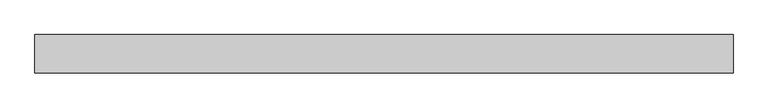
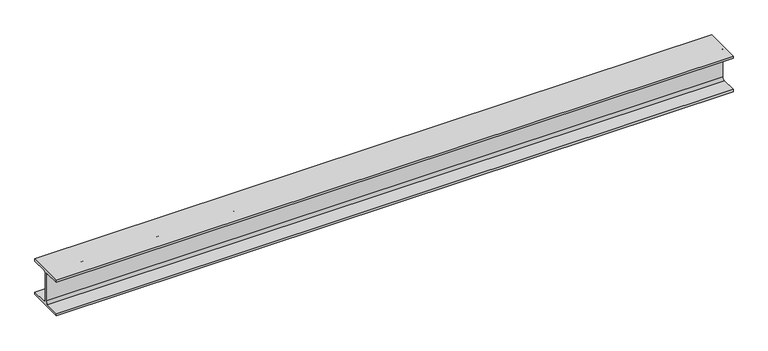
"""IFC4 building model written with IfcOpenShell, lengths in millimetres: beam geometry, 0912_Steel Framing_H-KSD3502 : H_SB_ASB_H-200x200x8x12."""

from ifc_helpers import new_model, si_unit, point, frame, frame_2d, origin, place, context, project, spatial, polyline, circle_curve, trimmed, segment, composite_curve, outline, extrude, source, transform, mapped, element, save


def beam_8723a7d4(model_context):
    return source(origin(), model_context, "Body", "SweptSolid", [
        extrude(outline(composite_curve([segment(polyline([(100.0, -88.0), (100.0, -100.0), (-100.0, -100.0), (-100.0, -88.0), (-17.0, -88.0)]), True, "CONTINUOUS"), segment(trimmed(circle_curve(frame_2d((-17.0, -75.0)), 13.0), [point((-17.0, -88.0))], [point((-4.0, -75.0))], True, "CARTESIAN"), True, "CONTINUOUS"), segment(polyline([(-4.0, -75.0), (-4.0, 75.0)]), True, "CONTINUOUS"), segment(trimmed(circle_curve(frame_2d((-17.0, 75.0)), 13.0), [point((-4.0, 75.0))], [point((-17.0, 88.0))], True, "CARTESIAN"), True, "CONTINUOUS"), segment(polyline([(-17.0, 88.0), (-100.0, 88.0), (-100.0, 100.0), (100.0, 100.0), (100.0, 88.0), (17.0, 88.0)]), True, "CONTINUOUS"), segment(trimmed(circle_curve(frame_2d((17.0, 75.0)), 13.0), [point((17.0, 88.0))], [point((4.0, 75.0))], True, "CARTESIAN"), True, "CONTINUOUS"), segment(polyline([(4.0, 75.0), (4.0, -75.0)]), True, "CONTINUOUS"), segment(trimmed(circle_curve(frame_2d((17.0, -75.0)), 13.0), [point((4.0, -75.0))], [point((17.0, -88.0))], True, "CARTESIAN"), True, "CONTINUOUS"), segment(polyline([(17.0, -88.0), (100.0, -88.0)]), True, "CONTINUOUS")], self_intersect=False)), frame((-1780.1436483, 0.0, 0.0), z_axis=(1.0, 0.0, 0.0), x_axis=(0.0, 1.0, 0.0)), (0.0, 0.0, 1.0), 3630.9979746),
    ])


if __name__ == "__main__":
    model = new_model("IFC4")
    model_context = context("Model", 3, world=origin())
    ifc_project = project(units=[si_unit("LENGTHUNIT", "METRE", prefix="MILLI")], contexts=[model_context])
    site = spatial("IfcSite", under=ifc_project)
    building = spatial("IfcBuilding", under=site)
    placement = place(None, origin())
    beam_shape = beam_8723a7d4(model_context)
    element("IfcBeam", 1, ObjectType="0912_Steel Framing_H-KSD3502 : H_SB_ASB_H-200x200x8x12", at=placement, inside=building, context=model_context, shape_type="MappedRepresentation", body=[
        mapped(beam_shape, transform((0.0, 0.0, 0.0), x_axis=(1.0, 0.0, 0.0), y_axis=(0.0, 1.0, 0.0), z_axis=(0.0, 0.0, 1.0))),
    ])
    save(model, "model.ifc")

# Revit data of these elements
# Type "0912_Steel Framing_H-KSD3502 : H_SB_ASB_H-200x200x8x12"
#   H_WM Code_1 = "S01AA002-00001 | Main Steel Structure Fabrication Work | Shelter/Building | Medium Steel - Standard (90KG/M>Weight≥30KG/M) | Material: (   )"
#   H_WM Code_2 = "S03AA028-00001 | Main Steel Structure Erection Work | Shelter/Building | Medium Steel (90KG/M>Weight≥30KG/M) | Material: (   )"
#   H_WM Code_3 = "S01AA010-00001 | Main Steel Structure Fabrication Work | Shelter/Building | Steel Painting/Coating | for Non-Fireproofed Steel Surface, Surface Preparation, Primer, Second & Final Coat | Material: (   )"
#   H_Q'ty Cal Type Tag = "SB-Q2"
#   Width = 20.0 cm
#   Web Thickness = 0.8 cm
#   Web Fillet = 1.3 cm
#   Warping Constant = 141000.0 cm⁶
#   W = 0
#   Torsional Moment of Inertia = 26.2485 cm⁴
#   Section Area = 63.53 cm²
#   Plastic Modulus weak axis = 244.0 cm³
#   Plastic Modulus strong axis = 525.0 cm³
#   Perimeter = 1.16 m²/m
#   Nominal Weight = 49.90 kgf/m
#   Moment of Inertia weak axis = 1600.00 cm⁴
#   Moment of Inertia strong axis = 4720.00 cm⁴
#   Height = 20.0 cm
#   Flange Thickness = 1.2 cm
#   Elastic Modulus weak axis = 160.0 cm³
#   Elastic Modulus strong axis = 472.0 cm³
#   Centroid Vertical = 10.0 cm
#   Centroid Horizontal = 10.0 cm
#   Ix = 47200000
#   Length [instance default] = 1.5240 m
#   Zx = 525000
#   b = 0.2000 m
#   h = 0.2000 m
#   r = 0.0130 m
#   s = 0.0080 m
#   t = 0.0120 m
#   A = 0.006353 m²
#   Structural Material [instance default] = Steel, 45-345
#   Assembly Code = ""
# Element 1 (IfcBeam, "0912_Steel Framing_H-KSD3502 : H_SB_ASB_H-200x200x8x12")
#   Structural Material = none
# Materials
#   "Steel, 45-345": class "Metal", colour RGB 189 187 185, transparency 0, Description = "Steel 345 MPa", Cost = 0
